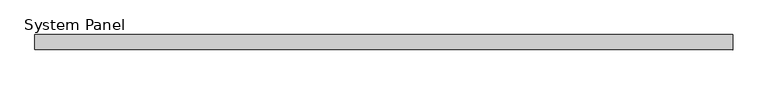
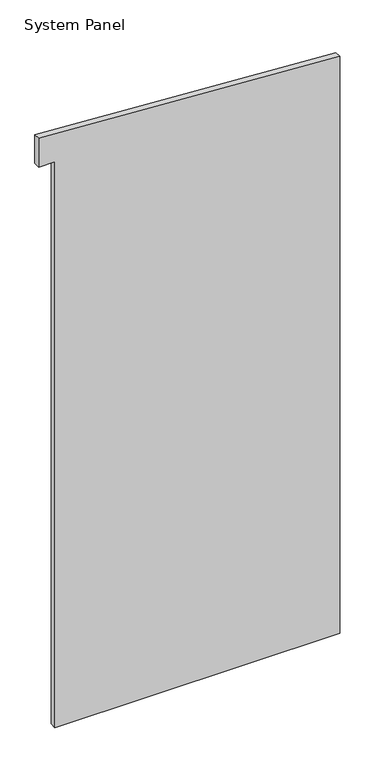
"""IFC4 building model written with IfcOpenShell, lengths in millimetres: plate geometry, System Panel : TEMPERED INSULATED GLAZING (CARDINAL GLASS LoĒ²-240."""

import ifcopenshell
import ifcopenshell.guid

model = None  # the IFC model being written
_history = None  # IfcOwnerHistory: only IFC2X3 demands one
_inside = {}  # id of a spatial element -> (the spatial element, [elements in it])
_under = {}  # id of a project, library or spatial element -> (it, [spatial elements below it])
_declared = {}  # id of a project -> (the project, [libraries it declares])
_typed = {}  # id of a type object -> (the type object, [elements of that type])
_made_of = {}  # id of a material, layer set ... -> (it, [elements and type objects made of it])


def new_model(schema):
    """Start an empty IFC model of exactly this schema.

    Asked for "IFC4X3", IfcOpenShell would pick the latest addendum, in which some entities
    have other attributes; the version numbers below select the first issue.
    IFC2X3 requires an IfcOwnerHistory on every rooted entity: one is made here for all.
    """
    global model, _history
    if schema == "IFC4X3":
        model = ifcopenshell.file(schema_version=(4, 3, 0, 0))
    else:
        model = ifcopenshell.file(schema=schema)
    _inside.clear()
    _under.clear()
    _declared.clear()
    _typed.clear()
    _made_of.clear()
    _history = None
    if model.schema == "IFC2X3":
        org = make("IfcOrganization", Name="unknown")
        user = make(
            "IfcPersonAndOrganization",
            ThePerson=make("IfcPerson", FamilyName="unknown"),
            TheOrganization=org,
        )
        app = make(
            "IfcApplication",
            ApplicationDeveloper=org,
            Version="unknown",
            ApplicationFullName="unknown",
            ApplicationIdentifier="unknown",
        )
        _history = make(
            "IfcOwnerHistory",
            OwningUser=user,
            OwningApplication=app,
            ChangeAction="ADDED",
            CreationDate=0,
        )
    return model


def make(cls, **values):
    """One entity of the class cls with the attributes given. An attribute that is None is left unset."""
    return model.create_entity(
        cls, **{name: value for name, value in values.items() if value is not None}
    )


def rooted(cls, **values):
    """An entity with a GlobalId (a new one), such as an element, a storey or a relation."""
    return make(cls, GlobalId=ifcopenshell.guid.new(), OwnerHistory=_history, **values)


def si_unit(unit_type, name, prefix=None):
    """IfcSIUnit, for example si_unit("LENGTHUNIT", "METRE", prefix="MILLI")."""
    return make("IfcSIUnit", UnitType=unit_type, Prefix=prefix, Name=name)


def assignment(units):
    """IfcUnitAssignment: the units of a project."""
    return None if units is None else make("IfcUnitAssignment", Units=units)


def point(xyz):
    """IfcCartesianPoint."""
    return None if xyz is None else make("IfcCartesianPoint", Coordinates=xyz)


def direction(xyz):
    """IfcDirection."""
    return None if xyz is None else make("IfcDirection", DirectionRatios=xyz)


def frame(location, z_axis=None, x_axis=None):
    """IfcAxis2Placement3D, a coordinate frame: its origin and axes. An axis left out is left unset."""
    return make(
        "IfcAxis2Placement3D",
        Location=point(location),
        Axis=direction(z_axis),
        RefDirection=direction(x_axis),
    )


def origin():
    """The frame at (0, 0, 0) with its axes left unset."""
    return frame((0.0, 0.0, 0.0))


def place(relative_to, where):
    """IfcLocalPlacement: puts the frame where relative to a parent placement (None: the world)."""
    return make(
        "IfcLocalPlacement", PlacementRelTo=relative_to, RelativePlacement=where
    )


def context(
    kind, dimensions, precision=None, world=None, true_north=None, identifier=None
):
    """IfcGeometricRepresentationContext, for example the 3D "Model" context."""
    return make(
        "IfcGeometricRepresentationContext",
        ContextIdentifier=identifier,
        ContextType=kind,
        CoordinateSpaceDimension=dimensions,
        Precision=precision,
        WorldCoordinateSystem=world,
        TrueNorth=true_north,
    )


def project(units=None, contexts=None):
    """IfcProject with its units and contexts."""
    return rooted(
        "IfcProject",
        Name="project",
        RepresentationContexts=contexts,
        UnitsInContext=assignment(units),
    )


def spatial(cls, under=None, at=None, **own):
    """A site, building, storey or space (cls), placed at a placement, below another one or the project."""
    s = rooted(cls, ObjectPlacement=at, **own)
    if under is not None:
        _under.setdefault(under.id(), (under, []))[1].append(s)
    return s


def polyline(points):
    """IfcPolyline through the points."""
    return make("IfcPolyline", Points=[point(p) for p in points])


def outline(outer, holes=None, kind="AREA"):
    """IfcArbitraryClosedProfileDef: a profile drawn as a closed curve; with holes, ...WithVoids."""
    if holes is None:
        return make("IfcArbitraryClosedProfileDef", ProfileType=kind, OuterCurve=outer)
    return make(
        "IfcArbitraryProfileDefWithVoids",
        ProfileType=kind,
        OuterCurve=outer,
        InnerCurves=holes,
    )


def extrude(swept, where, along, depth):
    """IfcExtrudedAreaSolid: the profile swept, set in the frame where, extruded along a direction by depth."""
    return make(
        "IfcExtrudedAreaSolid",
        SweptArea=swept,
        Position=where,
        ExtrudedDirection=direction(along),
        Depth=depth,
    )


def shape(context_of_items, identifier, shape_type, items):
    """IfcShapeRepresentation: the items that make up one representation, for example the "Body"."""
    return make(
        "IfcShapeRepresentation",
        ContextOfItems=context_of_items,
        RepresentationIdentifier=identifier,
        RepresentationType=shape_type,
        Items=items,
    )


def source(mapping_origin, context_of_items, identifier, shape_type, items):
    """IfcRepresentationMap: a shape defined once, which mapped items show again and again."""
    return make(
        "IfcRepresentationMap",
        MappingOrigin=mapping_origin,
        MappedRepresentation=shape(context_of_items, identifier, shape_type, items),
    )


def transform(
    local_origin,
    x_axis=None,
    y_axis=None,
    z_axis=None,
    scale=None,
    scale2=None,
    scale3=None,
    uniform=True,
):
    """IfcCartesianTransformationOperator3D, or its non-uniform kind. x_axis, y_axis, z_axis: its Axis1, 2, 3."""
    if uniform:
        return make(
            "IfcCartesianTransformationOperator3D",
            Axis1=direction(x_axis),
            Axis2=direction(y_axis),
            LocalOrigin=point(local_origin),
            Scale=scale,
            Axis3=direction(z_axis),
        )
    return make(
        "IfcCartesianTransformationOperator3DnonUniform",
        Axis1=direction(x_axis),
        Axis2=direction(y_axis),
        LocalOrigin=point(local_origin),
        Scale=scale,
        Axis3=direction(z_axis),
        Scale2=scale2,
        Scale3=scale3,
    )


def mapped(mapping_source, mapping_target):
    """IfcMappedItem: shows the shape of a source again, moved by a transform."""
    return make(
        "IfcMappedItem", MappingSource=mapping_source, MappingTarget=mapping_target
    )


def made_of(thing, what):
    """Note that an element or type object is made of a material, layer set ...; save() writes the relation."""
    if what is not None:
        _made_of.setdefault(what.id(), (what, []))[1].append(thing)
    return thing


def element(
    cls,
    number,
    at=None,
    inside=None,
    cuts=None,
    type_object=None,
    material=None,
    context=None,
    identifier="Body",
    shape_type=None,
    held_by="IfcProductDefinitionShape",
    body=None,
    shapes=None,
    **own,
):
    """One element of the class cls, such as IfcWall. Its Tag is "e" and its number.

    at: its placement. inside: the storey or other place that contains it. cuts: it is an
    opening in that element (IfcRelVoidsElement). A single representation is given by context,
    identifier, shape_type and body (its items); several are given by shapes. held_by: the class
    of the entity that holds the representations. save() writes the other relations.
    """
    e = rooted(cls, Tag="e%d" % number, ObjectPlacement=at, **own)
    if body is not None:
        shapes = [shape(context, identifier, shape_type, body)]
    if shapes is not None:
        e.Representation = make(held_by, Representations=shapes)
    if inside is not None:
        _inside.setdefault(inside.id(), (inside, []))[1].append(e)
    if cuts is not None:
        rooted(
            "IfcRelVoidsElement", RelatingBuildingElement=cuts, RelatedOpeningElement=e
        )
    if type_object is not None:
        _typed.setdefault(type_object.id(), (type_object, []))[1].append(e)
    return made_of(e, material)


def aggregate(whole, parts):
    """IfcRelAggregates: a whole, such as a stair, and the parts it consists of."""
    return rooted("IfcRelAggregates", RelatingObject=whole, RelatedObjects=parts)


def save(model, path):
    """Write the relations noted so far, then the file.

    IfcRelAggregates (storeys below a building ...), IfcRelContainedInSpatialStructure (elements
    in a storey), IfcRelDefinesByType, IfcRelAssociatesMaterial and IfcRelDeclares: one each for
    every whole, place, type object, material and project.
    """
    for whole, parts in _under.values():
        aggregate(whole, parts)
    for where, things in _inside.values():
        rooted(
            "IfcRelContainedInSpatialStructure",
            RelatedElements=things,
            RelatingStructure=where,
        )
    for kind, things in _typed.values():
        rooted("IfcRelDefinesByType", RelatedObjects=things, RelatingType=kind)
    for what, things in _made_of.values():
        rooted("IfcRelAssociatesMaterial", RelatedObjects=things, RelatingMaterial=what)
    for by, libraries in _declared.values():
        rooted("IfcRelDeclares", RelatingContext=by, RelatedDefinitions=libraries)
    model.write(path)


def system_panel_323ae763(model_context):
    return source(origin(), model_context, "Body", "SweptSolid", [
        extrude(outline(polyline([(0.0, -524.1120183), (0.0, 587.6120183), (2336.3357725, 587.6120183), (2381.4189069, 587.6120183), (2454.8704092, -587.6120183), (2336.3357725, -587.6120183), (2336.3357725, -524.1120183), (0.0, -524.1120183)])), frame((0.0, -31.75, 0.0), z_axis=(0.0, 1.0, 0.0), x_axis=(0.0, 0.0, 1.0)), (0.0, 0.0, 1.0), 25.4),
    ])


if __name__ == "__main__":
    model = new_model("IFC4")
    model_context = context("Model", 3, world=origin())
    ifc_project = project(units=[si_unit("LENGTHUNIT", "METRE", prefix="MILLI")], contexts=[model_context])
    site = spatial("IfcSite", under=ifc_project)
    building = spatial("IfcBuilding", under=site)
    placement = place(None, origin())
    system_panel_shape = system_panel_323ae763(model_context)
    element("IfcPlate", 1, ObjectType="System Panel : TEMPERED INSULATED GLAZING (CARDINAL GLASS LoĒ²-240", at=placement, inside=building, context=model_context, shape_type="MappedRepresentation", body=[
        mapped(system_panel_shape, transform((0.0, 0.0, 0.0), x_axis=(1.0, 0.0, 0.0), y_axis=(0.0, 1.0, 0.0), z_axis=(0.0, 0.0, 1.0))),
    ])
    save(model, "model.ifc")

# Revit data of these elements
# Type "System Panel : TEMPERED INSULATED GLAZING (CARDINAL GLASS LoĒ²-240"
#   Construction Type Id = "opn-s72"
#   Analytic Construction = "Double glazing - 1/4 in thick - low-E/clear (e = 0.1) glass"
#   Visual Light Transmittance = 0.72
#   Solar Heat Gain Coefficient = 0.6
#   Heat Transfer Coefficient (U) = 1.9873 W/(m²·K)
#   Transparency_Hack = 70
# Element 1 (IfcPlate, "System Panel : TEMPERED INSULATED GLAZING (CARDINAL GLASS LoĒ²-240")
#   Materials on its faces: "TEMPERED INSULATED GLAZING (CARDINAL GLASS LoĒ²-240\nOR EQUIVALENT)"
# Materials
#   "TEMPERED INSULATED GLAZING (CARDINAL GLASS LoĒ²-240\nOR EQUIVALENT)": class "Glass", colour RGB 196 205 210, transparency 0.85, Description = "Soda Lime Glass", Cost = 0
